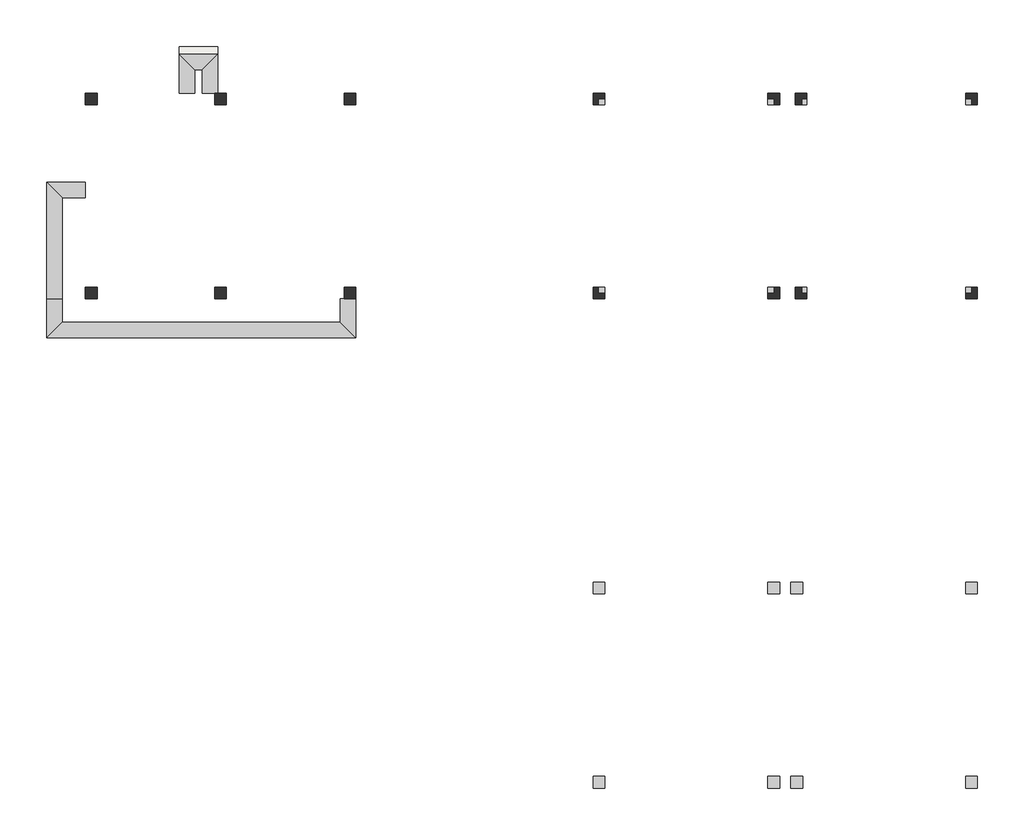
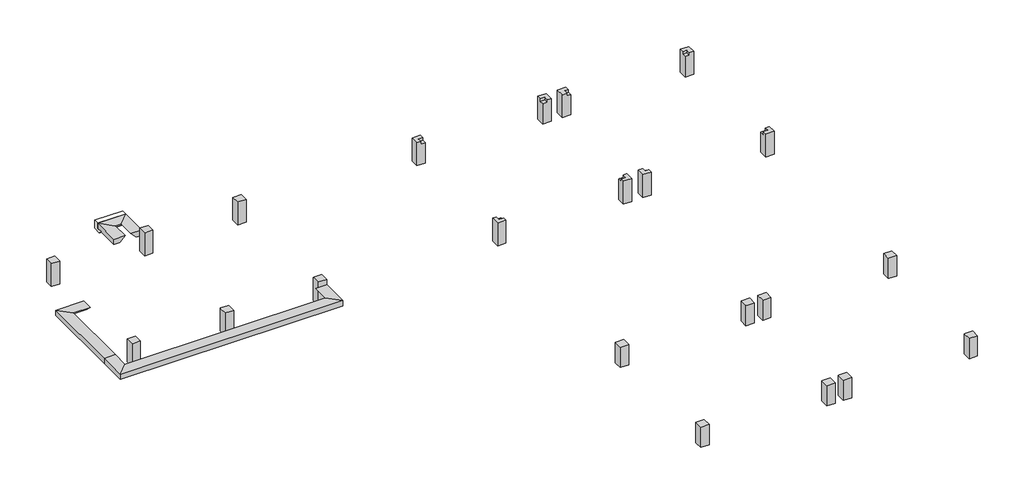
# One storey: 22 columns, 2 proxies, 1 slab.
"""IFC4 building model written with IfcOpenShell, lengths in millimetres."""

from ifc_helpers import new_model, si_unit, frame, origin, place, context, project, spatial, polyline, outline, extrude, faceted_brep, element, save

model = new_model("IFC4")

# Units and contexts
model_context = context("Model", 3, world=origin())
ifc_project = project(units=[si_unit("LENGTHUNIT", "METRE", prefix="MILLI")], contexts=[model_context])

# Site, building, storey
site = spatial("IfcSite", under=ifc_project)
building = spatial("IfcBuilding", under=site)
storey = spatial("IfcBuildingStorey", under=building, Name="T.O.C_-1,300", Elevation=-1300.0)

# Proxies
placement = place(None, origin())
element("IfcBuildingElementProxy", 1, Name="Slab Edge", ObjectType="Slab Edge", at=placement, inside=storey, context=model_context, shape_type="Brep", body=[
    faceted_brep([(10225.0, 13274.5208589, -600.0), (9925.0, 13274.5208589, -600.0), (9625.0, 13274.5208589, -300.0), (10225.0, 13274.5208589, -300.0), (10225.0, 11774.5208589, -300.0), (10225.0, 11774.5208589, -600.0), (9625.0, 12374.5208589, -300.0), (9925.0, 12074.5208589, -600.0), (-1725.0, 11774.5208589, -300.0), (-1725.0, 11774.5208589, -600.0), (-1125.0, 12374.5208589, -300.0), (-1425.0, 12074.5208589, -600.0), (-1725.0, 17774.5208589, -300.0), (-1725.0, 17774.5208589, -600.0), (-1725.0, 13274.5208589, -600.0), (-1725.0, 13274.5208589, -300.0), (-1125.0, 17174.5208589, -300.0), (-1125.0, 13274.5208589, -300.0), (-1425.0, 17474.5208589, -600.0), (-1425.0, 13274.5208589, -600.0), (-225.0, 17774.5208589, -600.0), (-225.0, 17774.5208589, -300.0), (-225.0, 17174.5208589, -300.0), (-225.0, 17474.5208589, -600.0)], [[[0, 1, 2, 3]], [[4, 5, 0, 3]], [[6, 4, 3, 2]], [[7, 6, 2, 1]], [[5, 7, 1, 0]], [[8, 9, 5, 4]], [[10, 8, 4, 6]], [[11, 10, 6, 7]], [[9, 11, 7, 5]], [[12, 13, 14, 15]], [[16, 12, 15, 17]], [[18, 16, 17, 19]], [[13, 18, 19, 14]], [[15, 14, 9, 8]], [[17, 15, 8, 10]], [[19, 17, 10, 11]], [[14, 19, 11, 9]], [[20, 21, 22, 23]], [[21, 20, 13, 12]], [[22, 21, 12, 16]], [[23, 22, 16, 18]], [[20, 23, 18, 13]]]),
])
element("IfcBuildingElementProxy", 2, Name="Slab Edge", ObjectType="Slab Edge", at=placement, inside=storey, context=model_context, shape_type="Brep", body=[
    faceted_brep([(4895.0, 21224.5208589, -450.0), (4895.0, 21224.5208589, -150.0), (4295.0, 21224.5208589, -150.0), (4595.0, 21224.5208589, -450.0), (4895.0, 22724.5208589, -450.0), (4895.0, 22724.5208589, -150.0), (4295.0, 22124.5208589, -150.0), (4595.0, 22424.5208589, -450.0), (3395.0, 22724.5208589, -450.0), (3395.0, 22724.5208589, -150.0), (3995.0, 22124.5208589, -150.0), (3695.0, 22424.5208589, -450.0), (3395.0, 21224.5208589, -450.0), (3695.0, 21224.5208589, -450.0), (3995.0, 21224.5208589, -150.0), (3395.0, 21224.5208589, -150.0)], [[[0, 1, 2, 3]], [[1, 0, 4, 5]], [[2, 1, 5, 6]], [[3, 2, 6, 7]], [[0, 3, 7, 4]], [[5, 4, 8, 9]], [[6, 5, 9, 10]], [[7, 6, 10, 11]], [[4, 7, 11, 8]], [[12, 13, 14, 15]], [[9, 8, 12, 15]], [[10, 9, 15, 14]], [[11, 10, 14, 13]], [[8, 11, 13, 12]]]),
])

# Columns
element("IfcColumn", 3, ObjectType="Concrete-Rectangular-Column : CL111_450x450", at=placement, inside=storey, context=model_context, shape_type="Brep", body=[
    faceted_brep([(225.0, 13724.5208589, -1300.0), (225.0, 13274.5208589, -1300.0), (-225.0, 13274.5208589, -1300.0), (-225.0, 13724.5208589, -1300.0), (225.0, 13724.5208589, 0.0), (225.0, 13674.5208589, 0.0), (225.0, 13274.5208589, 0.0), (225.0, 13274.5208589, -600.0), (-225.0, 13274.5208589, 0.0), (-225.0, 13724.5208589, 0.0), (-225.0, 13724.5208589, -600.0), (175.0, 13724.5208589, 0.0)], [[[0, 1, 2, 3]], [[4, 5, 6, 7, 1, 0]], [[6, 8, 2, 1, 7]], [[8, 9, 10, 3, 2]], [[9, 11, 4, 0, 3, 10]], [[4, 11, 9, 8, 6, 5]]]),
])
element("IfcColumn", 4, ObjectType="Concrete-Rectangular-Column : CL111_450x450", at=placement, inside=storey, context=model_context, shape_type="Brep", body=[
    faceted_brep([(5225.0, 13724.5208589, -1300.0), (5225.0, 13274.5208589, -1300.0), (4775.0, 13274.5208589, -1300.0), (4775.0, 13724.5208589, -1300.0), (5225.0, 13724.5208589, 0.0), (5225.0, 13674.5208589, 0.0), (5225.0, 13274.5208589, 0.0), (5225.0, 13274.5208589, -600.0), (4775.0, 13274.5208589, 0.0), (4775.0, 13274.5208589, -600.0), (4775.0, 13674.5208589, 0.0), (4775.0, 13724.5208589, 0.0)], [[[0, 1, 2, 3]], [[4, 5, 6, 7, 1, 0]], [[6, 8, 9, 2, 1, 7]], [[8, 10, 11, 3, 2, 9]], [[11, 4, 0, 3]], [[4, 11, 10, 8, 6, 5]]]),
])
element("IfcColumn", 5, ObjectType="Concrete-Rectangular-Column : CL111_450x450", at=placement, inside=storey, context=model_context, shape_type="Brep", body=[
    faceted_brep([(10225.0, 13724.5208589, -1300.0), (10225.0, 13274.5208589, -1300.0), (9775.0, 13274.5208589, -1300.0), (9775.0, 13724.5208589, -1300.0), (10225.0, 13724.5208589, 0.0), (10225.0, 13274.5208589, 0.0), (10225.0, 13724.5208589, -600.0), (9775.0, 13274.5208589, 0.0), (9775.0, 13274.5208589, -600.0), (9775.0, 13674.5208589, 0.0), (9775.0, 13724.5208589, 0.0), (9825.0, 13724.5208589, 0.0)], [[[0, 1, 2, 3]], [[4, 5, 1, 0, 6]], [[5, 7, 8, 2, 1]], [[7, 9, 10, 3, 2, 8]], [[10, 11, 4, 6, 0, 3]], [[4, 11, 10, 9, 7, 5]]]),
])
element("IfcColumn", 6, ObjectType="Concrete-Rectangular-Column : CL111_450x450", at=placement, inside=storey, context=model_context, shape_type="Brep", body=[
    faceted_brep([(10225.0, 21224.5208589, -1300.0), (10225.0, 20774.5208589, -1300.0), (9775.0, 20774.5208589, -1300.0), (9775.0, 21224.5208589, -1300.0), (10225.0, 21224.5208589, 0.0), (10225.0, 20774.5208589, 0.0), (10225.0, 20774.5208589, -600.0), (9825.0, 20774.5208589, 0.0), (9775.0, 20774.5208589, 0.0), (9775.0, 20824.5208589, 0.0), (9775.0, 21224.5208589, 0.0), (9775.0, 21224.5208589, -600.0)], [[[0, 1, 2, 3]], [[4, 5, 6, 1, 0]], [[5, 7, 8, 2, 1, 6]], [[8, 9, 10, 11, 3, 2]], [[10, 4, 0, 3, 11]], [[4, 10, 9, 8, 7, 5]]]),
])
element("IfcColumn", 7, ObjectType="Concrete-Rectangular-Column : CL111_450x450", at=placement, inside=storey, context=model_context, shape_type="Brep", body=[
    faceted_brep([(5225.0, 21224.5208589, -1300.0), (5225.0, 20774.5208589, -1300.0), (4775.0, 20774.5208589, -1300.0), (4775.0, 21224.5208589, -1300.0), (5225.0, 21224.5208589, 0.0), (5225.0, 20824.5208589, 0.0), (5225.0, 20774.5208589, 0.0), (5225.0, 21224.5208589, -600.0), (4775.0, 20774.5208589, 0.0), (4775.0, 21224.5208589, 0.0)], [[[0, 1, 2, 3]], [[4, 5, 6, 1, 0, 7]], [[6, 8, 2, 1]], [[8, 9, 3, 2]], [[9, 4, 7, 0, 3]], [[4, 9, 8, 6, 5]]]),
])
element("IfcColumn", 8, ObjectType="Concrete-Rectangular-Column : CL111_450x450", at=placement, inside=storey, context=model_context, shape_type="Brep", body=[
    faceted_brep([(225.0, 21224.5208589, -1300.0), (225.0, 20774.5208589, -1300.0), (-225.0, 20774.5208589, -1300.0), (-225.0, 21224.5208589, -1300.0), (225.0, 21224.5208589, 0.0), (225.0, 20824.5208589, 0.0), (225.0, 20774.5208589, 0.0), (225.0, 21224.5208589, -600.0), (175.0, 20774.5208589, 0.0), (-225.0, 20774.5208589, 0.0), (-225.0, 20774.5208589, -600.0), (-225.0, 21224.5208589, 0.0)], [[[0, 1, 2, 3]], [[4, 5, 6, 1, 0, 7]], [[6, 8, 9, 10, 2, 1]], [[9, 11, 3, 2, 10]], [[11, 4, 7, 0, 3]], [[4, 11, 9, 8, 6, 5]]]),
])
element("IfcColumn", 9, ObjectType="Concrete-Rectangular-Column : CL111_450x450", at=placement, inside=storey, context=model_context, shape_type="Brep", body=[
    faceted_brep([(26600.0, 13724.5208589, -1300.0), (26600.0, 13274.5208589, -1300.0), (26150.0, 13274.5208589, -1300.0), (26150.0, 13724.5208589, -1300.0), (26600.0, 13724.5208589, -600.0), (26600.0, 13724.5208589, 0.0), (26600.0, 13274.5208589, 0.0), (26150.0, 13274.5208589, 0.0), (26150.0, 13487.7731332, 0.0), (26150.0, 13487.7731332, -150.0), (26150.0, 13724.5208589, -150.0), (26200.0, 13724.5208589, -150.0), (26400.0, 13724.5208589, -150.0), (26400.0, 13724.5208589, 0.0), (26400.0, 13487.7731332, 0.0), (26400.0, 13487.7731332, -150.0)], [[[0, 1, 2, 3]], [[1, 0, 4, 5, 6]], [[2, 1, 6, 7]], [[3, 2, 7, 8, 9, 10]], [[0, 3, 10, 11, 12, 13, 5, 4]], [[6, 5, 13, 14, 8, 7]], [[9, 15, 12, 11, 10]], [[15, 14, 13, 12]], [[14, 15, 9, 8]]]),
])
element("IfcColumn", 10, ObjectType="Concrete-Rectangular-Column : CL111_450x450", at=placement, inside=storey, context=model_context, shape_type="Brep", body=[
    faceted_brep([(26600.0, 21224.5208589, -1300.0), (26600.0, 20774.5208589, -1300.0), (26150.0, 20774.5208589, -1300.0), (26150.0, 21224.5208589, -1300.0), (26600.0, 21224.5208589, 0.0), (26600.0, 20774.5208589, 0.0), (26600.0, 20774.5208589, -600.0), (26400.0, 20774.5208589, 0.0), (26400.0, 20774.5208589, -150.0), (26200.0, 20774.5208589, -150.0), (26150.0, 20774.5208589, -150.0), (26150.0, 20999.2709838, -150.0), (26150.0, 20999.2709838, 0.0), (26150.0, 21224.5208589, 0.0), (26400.0, 20999.2709838, 0.0), (26400.0, 20999.2709838, -150.0)], [[[0, 1, 2, 3]], [[1, 0, 4, 5, 6]], [[2, 1, 6, 5, 7, 8, 9, 10]], [[3, 2, 10, 11, 12, 13]], [[0, 3, 13, 4]], [[5, 4, 13, 12, 14, 7]], [[15, 11, 10, 9, 8]], [[14, 15, 8, 7]], [[15, 14, 12, 11]]]),
])
element("IfcColumn", 11, ObjectType="Concrete-Rectangular-Column : CL111_450x450", at=placement, inside=storey, context=model_context, shape_type="Brep", body=[
    faceted_brep([(27650.0, 13724.5208589, -1300.0), (27650.0, 13274.5208589, -1300.0), (27200.0, 13274.5208589, -1300.0), (27200.0, 13724.5208589, -1300.0), (27650.0, 13724.5208589, -600.0), (27650.0, 13724.5208589, -150.0), (27650.0, 13499.5208589, -150.0), (27650.0, 13499.5208589, 0.0), (27650.0, 13274.5208589, 0.0), (27200.0, 13274.5208589, 0.0), (27200.0, 13724.5208589, 0.0), (27250.0, 13724.5208589, 0.0), (27450.0, 13724.5208589, 0.0), (27450.0, 13724.5208589, -150.0), (27450.0, 13499.5208589, 0.0), (27450.0, 13499.5208589, -150.0)], [[[0, 1, 2, 3]], [[1, 0, 4, 5, 6, 7, 8]], [[2, 1, 8, 9]], [[3, 2, 9, 10]], [[0, 3, 10, 11, 12, 13, 5, 4]], [[9, 8, 7, 14, 12, 11, 10]], [[13, 15, 6, 5]], [[15, 14, 7, 6]], [[14, 15, 13, 12]]]),
])
element("IfcColumn", 12, ObjectType="Concrete-Rectangular-Column : CL111_450x450", at=placement, inside=storey, context=model_context, shape_type="Brep", body=[
    faceted_brep([(27650.0, 21224.5208589, -1300.0), (27650.0, 20774.5208589, -1300.0), (27200.0, 20774.5208589, -1300.0), (27200.0, 21224.5208589, -1300.0), (27650.0, 21224.5208589, 0.0), (27650.0, 20999.5208589, 0.0), (27650.0, 20999.5208589, -150.0), (27650.0, 20774.5208589, -150.0), (27650.0, 20774.5208589, -600.0), (27450.0, 20774.5208589, -150.0), (27450.0, 20774.5208589, 0.0), (27250.0, 20774.5208589, 0.0), (27200.0, 20774.5208589, 0.0), (27200.0, 21224.5208589, 0.0), (27450.0, 20999.5208589, 0.0), (27450.0, 20999.5208589, -150.0)], [[[0, 1, 2, 3]], [[1, 0, 4, 5, 6, 7, 8]], [[2, 1, 8, 7, 9, 10, 11, 12]], [[3, 2, 12, 13]], [[0, 3, 13, 4]], [[13, 12, 11, 10, 14, 5, 4]], [[6, 15, 9, 7]], [[15, 14, 10, 9]], [[14, 15, 6, 5]]]),
])
element("IfcColumn", 13, ObjectType="Concrete-Rectangular-Column : CL111_450x450", at=placement, inside=storey, context=model_context, shape_type="Brep", body=[
    faceted_brep([(34245.0, 13724.5208589, -1300.0), (34245.0, 13274.5208589, -1300.0), (33795.0, 13274.5208589, -1300.0), (33795.0, 13724.5208589, -1300.0), (34245.0, 13724.5208589, -600.0), (34245.0, 13724.5208589, 0.0), (34245.0, 13274.5208589, 0.0), (33795.0, 13274.5208589, 0.0), (33795.0, 13499.5208589, 0.0), (33795.0, 13499.5208589, -150.0), (33795.0, 13724.5208589, -150.0), (33845.0, 13724.5208589, -150.0), (34020.0, 13724.5208589, -150.0), (34020.0, 13724.5208589, 0.0), (34020.0, 13499.5208589, 0.0), (34020.0, 13499.5208589, -150.0)], [[[0, 1, 2, 3]], [[1, 0, 4, 5, 6]], [[2, 1, 6, 7]], [[3, 2, 7, 8, 9, 10]], [[0, 3, 10, 11, 12, 13, 5, 4]], [[6, 5, 13, 14, 8, 7]], [[9, 15, 12, 11, 10]], [[15, 14, 13, 12]], [[14, 15, 9, 8]]]),
])
element("IfcColumn", 14, ObjectType="Concrete-Rectangular-Column : CL111_450x450", at=placement, inside=storey, context=model_context, shape_type="Brep", body=[
    faceted_brep([(34245.0, 21224.5208589, -1300.0), (34245.0, 20774.5208589, -1300.0), (33795.0, 20774.5208589, -1300.0), (33795.0, 21224.5208589, -1300.0), (34245.0, 21224.5208589, 0.0), (34245.0, 20774.5208589, 0.0), (34245.0, 20774.5208589, -600.0), (34020.0, 20774.5208589, 0.0), (34020.0, 20774.5208589, -150.0), (33845.0, 20774.5208589, -150.0), (33795.0, 20774.5208589, -150.0), (33795.0, 20999.5208589, -150.0), (33795.0, 20999.5208589, 0.0), (33795.0, 21224.5208589, 0.0), (34020.0, 20999.5208589, 0.0), (34020.0, 20999.5208589, -150.0)], [[[0, 1, 2, 3]], [[1, 0, 4, 5, 6]], [[2, 1, 6, 5, 7, 8, 9, 10]], [[3, 2, 10, 11, 12, 13]], [[0, 3, 13, 4]], [[5, 4, 13, 12, 14, 7]], [[15, 11, 10, 9, 8]], [[14, 15, 8, 7]], [[15, 14, 12, 11]]]),
])
element("IfcColumn", 15, ObjectType="Concrete-Rectangular-Column : CL111_450x450", at=placement, inside=storey, context=model_context, shape_type="Brep", body=[
    faceted_brep([(19395.0, 13274.5208589, -1300.0), (19395.0, 13724.5208589, -1300.0), (19845.0, 13724.5208589, -1300.0), (19845.0, 13274.5208589, -1300.0), (19395.0, 13274.5208589, 0.0), (19395.0, 13724.5208589, 0.0), (19395.0, 13724.5208589, -600.0), (19845.0, 13274.5208589, 0.0), (19845.0, 13724.5208589, -150.0), (19845.0, 13487.7731332, -150.0), (19845.0, 13487.7731332, 0.0), (19595.0, 13724.5208589, 0.0), (19595.0, 13724.5208589, -150.0), (19795.0, 13724.5208589, -150.0), (19595.0, 13487.7731332, 0.0), (19595.0, 13487.7731332, -150.0)], [[[0, 1, 2, 3]], [[1, 0, 4, 5, 6]], [[0, 3, 7, 4]], [[3, 2, 8, 9, 10, 7]], [[2, 1, 6, 5, 11, 12, 13, 8]], [[5, 4, 7, 10, 14, 11]], [[12, 15, 9, 8, 13]], [[15, 14, 10, 9]], [[14, 15, 12, 11]]]),
])
element("IfcColumn", 16, ObjectType="Concrete-Rectangular-Column : CL111_450x450", at=placement, inside=storey, context=model_context, shape_type="Brep", body=[
    faceted_brep([(19395.0, 20774.5208589, -1300.0), (19395.0, 21224.5208589, -1300.0), (19845.0, 21224.5208589, -1300.0), (19845.0, 20774.5208589, -1300.0), (19395.0, 20774.5208589, -600.0), (19395.0, 20774.5208589, 0.0), (19395.0, 21224.5208589, 0.0), (19845.0, 20774.5208589, -150.0), (19795.0, 20774.5208589, -150.0), (19595.0, 20774.5208589, -150.0), (19595.0, 20774.5208589, 0.0), (19845.0, 21224.5208589, 0.0), (19845.0, 20999.2709838, 0.0), (19845.0, 20999.2709838, -150.0), (19595.0, 20999.2709838, 0.0), (19595.0, 20999.2709838, -150.0)], [[[0, 1, 2, 3]], [[1, 0, 4, 5, 6]], [[0, 3, 7, 8, 9, 10, 5, 4]], [[3, 2, 11, 12, 13, 7]], [[2, 1, 6, 11]], [[6, 5, 10, 14, 12, 11]], [[13, 15, 9, 8, 7]], [[15, 14, 10, 9]], [[14, 15, 13, 12]]]),
])
element("IfcColumn", 17, ObjectType="Concrete-Rectangular-Column : CL111_450x450", at=placement, inside=storey, context=model_context, shape_type="Brep", body=[
    faceted_brep([(26600.0, -5175.4791411, -1300.0), (26600.0, -5625.4791411, -1300.0), (26150.0, -5625.4791411, -1300.0), (26150.0, -5175.4791411, -1300.0), (26600.0, -5175.4791411, -600.0), (26600.0, -5175.4791411, -150.0), (26600.0, -5625.4791411, -150.0), (26150.0, -5625.4791411, -150.0), (26150.0, -5175.4791411, -150.0), (26200.0, -5175.4791411, -150.0)], [[[0, 1, 2, 3]], [[1, 0, 4, 5, 6]], [[2, 1, 6, 7]], [[3, 2, 7, 8]], [[0, 3, 8, 9, 5, 4]], [[6, 5, 9, 8, 7]]]),
])
element("IfcColumn", 18, ObjectType="Concrete-Rectangular-Column : CL111_450x450", at=placement, inside=storey, context=model_context, shape_type="Brep", body=[
    faceted_brep([(26600.0, 2324.5208589, -1300.0), (26600.0, 1874.5208589, -1300.0), (26150.0, 1874.5208589, -1300.0), (26150.0, 2324.5208589, -1300.0), (26600.0, 2324.5208589, -150.0), (26600.0, 1874.5208589, -150.0), (26600.0, 1874.5208589, -600.0), (26200.0, 1874.5208589, -150.0), (26150.0, 1874.5208589, -150.0), (26150.0, 2324.5208589, -150.0)], [[[0, 1, 2, 3]], [[1, 0, 4, 5, 6]], [[2, 1, 6, 5, 7, 8]], [[3, 2, 8, 9]], [[0, 3, 9, 4]], [[5, 4, 9, 8, 7]]]),
])
element("IfcColumn", 19, ObjectType="Concrete-Rectangular-Column : CL111_450x450", at=placement, inside=storey, context=model_context, shape_type="Brep", body=[
    faceted_brep([(27490.0, -5175.4791411, -1300.0), (27490.0, -5625.4791411, -1300.0), (27040.0, -5625.4791411, -1300.0), (27040.0, -5175.4791411, -1300.0), (27490.0, -5175.4791411, -600.0), (27490.0, -5175.4791411, -150.0), (27490.0, -5625.4791411, -150.0), (27040.0, -5625.4791411, -150.0), (27040.0, -5175.4791411, -150.0), (27090.0, -5175.4791411, -150.0)], [[[0, 1, 2, 3]], [[1, 0, 4, 5, 6]], [[2, 1, 6, 7]], [[3, 2, 7, 8]], [[0, 3, 8, 9, 5, 4]], [[6, 5, 9, 8, 7]]]),
])
element("IfcColumn", 20, ObjectType="Concrete-Rectangular-Column : CL111_450x450", at=placement, inside=storey, context=model_context, shape_type="Brep", body=[
    faceted_brep([(27490.0, 2324.5208589, -1300.0), (27490.0, 1874.5208589, -1300.0), (27040.0, 1874.5208589, -1300.0), (27040.0, 2324.5208589, -1300.0), (27490.0, 2324.5208589, -150.0), (27490.0, 1874.5208589, -150.0), (27490.0, 1874.5208589, -600.0), (27090.0, 1874.5208589, -150.0), (27040.0, 1874.5208589, -150.0), (27040.0, 2324.5208589, -150.0)], [[[0, 1, 2, 3]], [[1, 0, 4, 5, 6]], [[2, 1, 6, 5, 7, 8]], [[3, 2, 8, 9]], [[0, 3, 9, 4]], [[5, 4, 9, 8, 7]]]),
])
element("IfcColumn", 21, ObjectType="Concrete-Rectangular-Column : CL111_450x450", at=placement, inside=storey, context=model_context, shape_type="Brep", body=[
    faceted_brep([(34245.0, -5175.4791411, -1300.0), (34245.0, -5625.4791411, -1300.0), (33795.0, -5625.4791411, -1300.0), (33795.0, -5175.4791411, -1300.0), (34245.0, -5175.4791411, -600.0), (34245.0, -5175.4791411, -150.0), (34245.0, -5625.4791411, -150.0), (33795.0, -5625.4791411, -150.0), (33795.0, -5175.4791411, -150.0), (33845.0, -5175.4791411, -150.0)], [[[0, 1, 2, 3]], [[1, 0, 4, 5, 6]], [[2, 1, 6, 7]], [[3, 2, 7, 8]], [[0, 3, 8, 9, 5, 4]], [[6, 5, 9, 8, 7]]]),
])
element("IfcColumn", 22, ObjectType="Concrete-Rectangular-Column : CL111_450x450", at=placement, inside=storey, context=model_context, shape_type="Brep", body=[
    faceted_brep([(34245.0, 2324.5208589, -1300.0), (34245.0, 1874.5208589, -1300.0), (33795.0, 1874.5208589, -1300.0), (33795.0, 2324.5208589, -1300.0), (34245.0, 2324.5208589, -150.0), (34245.0, 1874.5208589, -150.0), (34245.0, 1874.5208589, -600.0), (33845.0, 1874.5208589, -150.0), (33795.0, 1874.5208589, -150.0), (33795.0, 2324.5208589, -150.0)], [[[0, 1, 2, 3]], [[1, 0, 4, 5, 6]], [[2, 1, 6, 5, 7, 8]], [[3, 2, 8, 9]], [[0, 3, 9, 4]], [[5, 4, 9, 8, 7]]]),
])
element("IfcColumn", 23, ObjectType="Concrete-Rectangular-Column : CL111_450x450", at=placement, inside=storey, context=model_context, shape_type="Brep", body=[
    faceted_brep([(19395.0, -5625.4791411, -1300.0), (19395.0, -5175.4791411, -1300.0), (19845.0, -5175.4791411, -1300.0), (19845.0, -5625.4791411, -1300.0), (19395.0, -5625.4791411, -150.0), (19395.0, -5175.4791411, -150.0), (19395.0, -5175.4791411, -600.0), (19845.0, -5625.4791411, -150.0), (19845.0, -5175.4791411, -150.0), (19795.0, -5175.4791411, -150.0)], [[[0, 1, 2, 3]], [[1, 0, 4, 5, 6]], [[0, 3, 7, 4]], [[3, 2, 8, 7]], [[2, 1, 6, 5, 9, 8]], [[5, 4, 7, 8, 9]]]),
])
element("IfcColumn", 24, ObjectType="Concrete-Rectangular-Column : CL111_450x450", at=placement, inside=storey, context=model_context, shape_type="Brep", body=[
    faceted_brep([(19395.0, 1874.5208589, -1300.0), (19395.0, 2324.5208589, -1300.0), (19845.0, 2324.5208589, -1300.0), (19845.0, 1874.5208589, -1300.0), (19395.0, 1874.5208589, -600.0), (19395.0, 1874.5208589, -150.0), (19395.0, 2324.5208589, -150.0), (19845.0, 1874.5208589, -150.0), (19795.0, 1874.5208589, -150.0), (19845.0, 2324.5208589, -150.0)], [[[0, 1, 2, 3]], [[1, 0, 4, 5, 6]], [[0, 3, 7, 8, 5, 4]], [[3, 2, 9, 7]], [[2, 1, 6, 9]], [[6, 5, 8, 7, 9]]]),
])

# Slab
element("IfcSlab", 25, ObjectType="STOOP_SLAB EDGE(계단부분) : STOOP_SLAB EDGE(계단부분)", at=placement, inside=storey, context=model_context, shape_type="SweptSolid", body=[
    extrude(outline(polyline([(23024.5208589, -150.0), (23024.5208589, -600.0), (22574.5208589, -600.0), (22424.5208589, -450.0), (22724.5208589, -450.0), (22724.5208589, -150.0), (23024.5208589, -150.0)])), frame((3393.3757722, 0.0, 0.0), z_axis=(1.0, 0.0, 0.0), x_axis=(0.0, 1.0, 0.0)), (0.0, 0.0, 1.0), 1501.6242278),
])

save(model, "model.ifc")

# Revit data of these elements
# Type "Concrete-Rectangular-Column : CL111_450x450"
#   Description = "UG 철골 기둥용 Pedestal"
#   b = 450 mm
#   h = 450 mm
#   hec_material3 [instance default] = none
#   hec_material2 [instance default] = A03AE056-00001_Bitumen/Bituminous/Asphalt Coating
#   hec_material1 [instance default] = A03AC035-00001_Form Work (3 times in use)_Flat
#   Structural Material [instance default] = A03AC032-00007_Structural Concrete_Type1_25MPa-30Mpa
# Type "STOOP_SLAB EDGE(계단부분) : STOOP_SLAB EDGE(계단부분)"
#   built-in parameter 1001306 [instance default] = 3.93701 (stored number, unit not read)
#   Default Elevation = 0
#   Structural Material = none
# Elements 1, 2 (IfcBuildingElementProxy, "Slab Edge")
#   W11) Activity ID = "C02AGB040"
#   W12) Activity Name = "Main Gate Security Building ‐ Exterior & Finish Work"
#   W13) Plan Start Date = "2017-01-12"
#   W14) Plan Finish Date = "2017-04-11"
#   W15) Duration = "71"
#   W16) Actual Start Date = "2017-01-12"
#   W17) Actual Finish Date = "2017-04-11"
#   Phase Created = New Construction
#   Materials on its faces: "A03AD032-00007_Structural Concrete_25MPa-30MPa"
# Elements 3, 4, 5, 6, 7, 9, 10, 11, 12, 13, 14, 15, 16, 17, 18, 19, 20, 21, 22, 23, 24 (IfcColumn, "Concrete-Rectangular-Column : CL111_450x450")
#   Comments = ""
#   F01) Building Name = "Main Gate House"
#   F11) Project Building Tag_Type-1 = "Common"
#   F12) Project Building Tag_Type-2 = "Common"
#   F13) Project Facility Code = "Facility Code"
#   F21) Structural Type = "Concrete"
#   F31) Standard Building Code = "IBC"
#   F41) Discipline = "AR"
#   F51) Plan Start Date-Engineering = "2015-01-01"
#   F52) Plan Finish Date-Engineering = "2015-12-31"
#   F53) Duration = "365"
#   F54) Actual Start Date-Engineering = "2015-01-01"
#   F55) Actual Finish Date-Engineering = "2015-12-31"
#   F61) Plan Start Date-Construction = "2016-08-19"
#   F62) Plan Finish Date-Construction = "2017-01-31"
#   F64) Actual Start Date-Construction = "2016-08-19"
#   F63) Duration = "202"
#   F65) Actual Finish Date-Construction = "2017-01-31"
#   F91) Plant Type = "CFPP"
#   F92) KKS Structures, Building = "UYF"
#   P01) Project Name = "TVEP"
#   P02) Project Configuration = "CFB Boiler x 2(Foster Wheeler) + STG x 2(Alstom, 150MW)"
#   P03) Project Abbreviation = "TVEP"
#   P04) Project Code = "BEPH1402"
#   P05) Project Stage = "In operation"
#   P06) Project Location = "Sito Looc, Barangay Bato, Toledo City in Philippines"
#   P07) Project Owner = "Therma Visayas, Inc."
#   P08) Project O.E = "Flour"
#   P09) Project Schedule = "ITB Issueing Date : 2013.07.30\r\nSite Survey : 2013.08.19-20\r\nBid Closing Date : 2013.11.29\r\nPreferred Bidder Notice 접수 : 2014.04.27\r\nTarget award date : 2014 05\r\nLOA 접수 : 2014.05.21\r\nSigning Ceremony : 2014.05.30"
#   P10) Basic Wind Speed = "55.6 m/s"
#   P11) Seismic = "NSCP 2010, Zone 4 (PGA : 0.4g)"
#   P12) Soil = "Sc"
#   P13) Soil Capacity = "100kN/m2"
#   P14) Pile Capacity = "PHC(D400) : 1200kN"
#   W00) Work Master Code = "A03AC032-00007"
#   W01) Work Master_Lv1 = "Concrete Work"
#   W02) Work Master_Lv2 = "Substructure Work"
#   W03) Work Master_Spec.1 = "Structural Concrete"
#   W04) Work Master_Spec.2 = "Cement Type-1"
#   W05) Work Master_Spec.3 = "25MPa < F'c (Cylinder Strength) ≤ 30MPa"
#   W11) Activity ID = "C02AGB010"
#   W12) Activity Name = "Main Gate Security Building ‐ Building Foundaton"
#   W13) Plan Start Date = "2016-08-19"
#   W14) Plan Finish Date = "2016-09-22"
#   W15) Duration = "26"
#   W16) Actual Start Date = "2016-08-19"
#   W17) Actual Finish Date = "2016-09-22"
#   R02) Unit Price = 0
#   Structural Material = A03AD032-00007_Structural Concrete_25MPa-30MPa
#   hec_material3 = none
#   hec_material2 = none
#   hec_material1 = none
#   Phase Created = New Construction
#   Materials on its faces: "A03AD032-00007_Structural Concrete_25MPa-30MPa"
# Element 8 (IfcColumn, "Concrete-Rectangular-Column : CL111_450x450")
#   Comments = ""
#   F01) Building Name = "Main Gate House"
#   F11) Project Building Tag_Type-1 = "Common"
#   F12) Project Building Tag_Type-2 = "Common"
#   F13) Project Facility Code = "Facility Code"
#   F21) Structural Type = "Concrete"
#   F31) Standard Building Code = "IBC"
#   F41) Discipline = "AR"
#   F51) Plan Start Date-Engineering = "2015-01-01"
#   F52) Plan Finish Date-Engineering = "2015-12-31"
#   F53) Duration = "365"
#   F54) Actual Start Date-Engineering = "2015-01-01"
#   F55) Actual Finish Date-Engineering = "2015-12-31"
#   F61) Plan Start Date-Construction = "2016-08-19"
#   F62) Plan Finish Date-Construction = "2017-01-31"
#   F64) Actual Start Date-Construction = "2016-08-19"
#   F63) Duration = "202"
#   F65) Actual Finish Date-Construction = "2017-01-31"
#   F91) Plant Type = "CFPP"
#   F92) KKS Structures, Building = "UYF"
#   P01) Project Name = "TVEP"
#   P02) Project Configuration = "CFB Boiler x 2(Foster Wheeler) + STG x 2(Alstom, 150MW)"
#   P03) Project Abbreviation = "TVEP"
#   P04) Project Code = "BEPH1402"
#   P05) Project Stage = "In operation"
#   P06) Project Location = "Sito Looc, Barangay Bato, Toledo City in Philippines"
#   P07) Project Owner = "Therma Visayas, Inc."
#   P08) Project O.E = "Flour"
#   P09) Project Schedule = "ITB Issueing Date : 2013.07.30\r\nSite Survey : 2013.08.19-20\r\nBid Closing Date : 2013.11.29\r\nPreferred Bidder Notice 접수 : 2014.04.27\r\nTarget award date : 2014 05\r\nLOA 접수 : 2014.05.21\r\nSigning Ceremony : 2014.05.30"
#   P10) Basic Wind Speed = "55.6 m/s"
#   P11) Seismic = "NSCP 2010, Zone 4 (PGA : 0.4g)"
#   P12) Soil = "Sc"
#   P13) Soil Capacity = "100kN/m2"
#   P14) Pile Capacity = "PHC(D400) : 1200kN"
#   W00) Work Master Code = "A03AC032-00007"
#   W01) Work Master_Lv1 = "Concrete Work"
#   W02) Work Master_Lv2 = "Substructure Work"
#   W03) Work Master_Spec.1 = "Structural Concrete"
#   W04) Work Master_Spec.2 = "Cement Type-1"
#   W05) Work Master_Spec.3 = "25MPa < F'c (Cylinder Strength) ≤ 30MPa"
#   W11) Activity ID = "C02AGB010"
#   W12) Activity Name = "Main Gate Security Building ‐ Building Foundaton"
#   W13) Plan Start Date = "2016-08-19"
#   W14) Plan Finish Date = "2016-09-22"
#   W15) Duration = "26"
#   W16) Actual Start Date = "2016-08-19"
#   W17) Actual Finish Date = "2016-09-22"
#   TMP_Element Name = "C1"
#   R02) Unit Price = 0
#   Structural Material = A03AD032-00007_Structural Concrete_25MPa-30MPa
#   hec_material3 = none
#   hec_material2 = none
#   hec_material1 = none
#   Phase Created = New Construction
#   Materials on its faces: "A03AD032-00007_Structural Concrete_25MPa-30MPa"
# Element 25 (IfcSlab, "STOOP_SLAB EDGE(계단부분) : STOOP_SLAB EDGE(계단부분)")
#   F01) Building Name = "Main Gate House"
#   F11) Project Building Tag_Type-1 = "Common"
#   F12) Project Building Tag_Type-2 = "Common"
#   F13) Project Facility Code = "Facility Code"
#   F21) Structural Type = "Concrete"
#   F31) Standard Building Code = "IBC"
#   F41) Discipline = "AR"
#   F51) Plan Start Date-Engineering = "2015-01-01"
#   F52) Plan Finish Date-Engineering = "2015-12-31"
#   F53) Duration = "365"
#   F54) Actual Start Date-Engineering = "2015-01-01"
#   F55) Actual Finish Date-Engineering = "2015-12-31"
#   F61) Plan Start Date-Construction = "2016-08-19"
#   F62) Plan Finish Date-Construction = "2017-01-31"
#   F64) Actual Start Date-Construction = "2016-08-19"
#   F63) Duration = "202"
#   F65) Actual Finish Date-Construction = "2017-01-31"
#   F91) Plant Type = "CFPP"
#   F92) KKS Structures, Building = "UYF"
#   P01) Project Name = "TVEP"
#   P02) Project Configuration = "CFB Boiler x 2(Foster Wheeler) + STG x 2(Alstom, 150MW)"
#   P03) Project Abbreviation = "TVEP"
#   P04) Project Code = "BEPH1402"
#   P05) Project Stage = "In operation"
#   P06) Project Location = "Sito Looc, Barangay Bato, Toledo City in Philippines"
#   P07) Project Owner = "Therma Visayas, Inc."
#   P08) Project O.E = "Flour"
#   P09) Project Schedule = "ITB Issueing Date : 2013.07.30\r\nSite Survey : 2013.08.19-20\r\nBid Closing Date : 2013.11.29\r\nPreferred Bidder Notice 접수 : 2014.04.27\r\nTarget award date : 2014 05\r\nLOA 접수 : 2014.05.21\r\nSigning Ceremony : 2014.05.30"
#   P10) Basic Wind Speed = "55.6 m/s"
#   P11) Seismic = "NSCP 2010, Zone 4 (PGA : 0.4g)"
#   P12) Soil = "Sc"
#   P13) Soil Capacity = "100kN/m2"
#   P14) Pile Capacity = "PHC(D400) : 1200kN"
#   W11) Activity ID = "C02AGB040"
#   W12) Activity Name = "Main Gate Security Building ‐ Exterior & Finish Work"
#   W13) Plan Start Date = "2017-01-12"
#   W14) Plan Finish Date = "2017-04-11"
#   W15) Duration = "71"
#   W16) Actual Start Date = "2017-01-12"
#   W17) Actual Finish Date = "2017-04-11"
#   R02) Unit Price = 0
#   built-in parameter 1001306 = 4.92659 (stored number, unit not read)
#   Phase Created = New Construction
# Materials
#   "A03AE056-00001_Bitumen/Bituminous/Asphalt Coating": class "Generic", colour RGB 17 17 17, transparency 0, Description = "Damp-proofing", W00) Work Master Code = "A03AE056-00001", W01) Work Master_Lv1 = "Concrete Work", W02) Work Master_Lv2 = "Concrete Protective Coating (U/G)", W03) Work Master_Spec.1 = "Bitumen/Bituminous/Asphalt Coating", Cost = 0
#   "A03AC035-00001_Form Work (3 times in use)_Flat": class "Wood", colour RGB 149 120 74, transparency 0, Description = "Plywood", W00) Work Master Code = "A03AC035-00001", W01) Work Master_Lv1 = "Concrete Work", W02) Work Master_Lv2 = "Substructure Work", W03) Work Master_Spec.1 = "Form Work (3 times in use)", W04) Work Master_Spec.2 = "Flat Form", W05) Work Master_Spec.3 = "Dressed Lumber, Plywood or Steel Form(Wood Planks are not Allowed) incl. Chamfer", Cost = 0
#   "A03AC032-00007_Structural Concrete_Type1_25MPa-30Mpa": class "Concrete", colour RGB 176 176 176, transparency 0, Keynote = "09910.A1", Description = "Reinf. Conc.", W00) Work Master Code = "A03AC032-00007", W01) Work Master_Lv1 = "Concrete Work", W02) Work Master_Lv2 = "Substructure Work", W03) Work Master_Spec.1 = "Structural Concrete", W04) Work Master_Spec.2 = "Cement Type-1", W05) Work Master_Spec.3 = "25MPa < F'c (Cylinder Strength) ≤ 30MPa", Cost = 0
#   "A03AD032-00007_Structural Concrete_25MPa-30MPa": class "Concrete", colour RGB 176 176 176, transparency 0, Keynote = "09910.A1", Description = "Reinf. Conc.", W00) Work Master Code = "A03AD032-00007", W01) Work Master_Lv1 = "Concrete Work", W02) Work Master_Lv2 = "Superstructure Work", W03) Work Master_Spec.1 = "Structural Concrete", W04) Work Master_Spec.2 = "Cement Type-1", W05) Work Master_Spec.3 = "25MPa < F'c (Cylinder Strength) ≤ 30MPa", Cost = 0
# Room, not placed, phase "New Construction", upper offset 0 mm, lower offset 0 mm
#   Comments = ""
#   Base Finish = "EXPOXY PAINT ON THK.15 CEMENT PLASTER(H=100)"
#   Ceiling Finish = "LATEX PAINT ON FAIR FACED CONC."
#   Wall Finish = "LATEX PAINT ON THK.15 CEMENT PLASTER + MASONRY WALL"
#   Floor Finish = "EPOXY PAINT ON STEEL TROWELED CONC. SLAB"
#   Number = "1"
#   Name = ""
#   F01) Building Name = "CENTRAL CONTROL BUILDING"
#   S01) Room Name = "CABLE ROOM"
#   S02) Room Number(Project) = "UCA01R0001"
# Room, not placed, phase "New Construction", upper offset 0 mm, lower offset 0 mm
#   Comments = ""
#   Number = "2"
#   Name = ""
#   S01) Room Name = ""
#   S02) Room Number(Project) = ""
